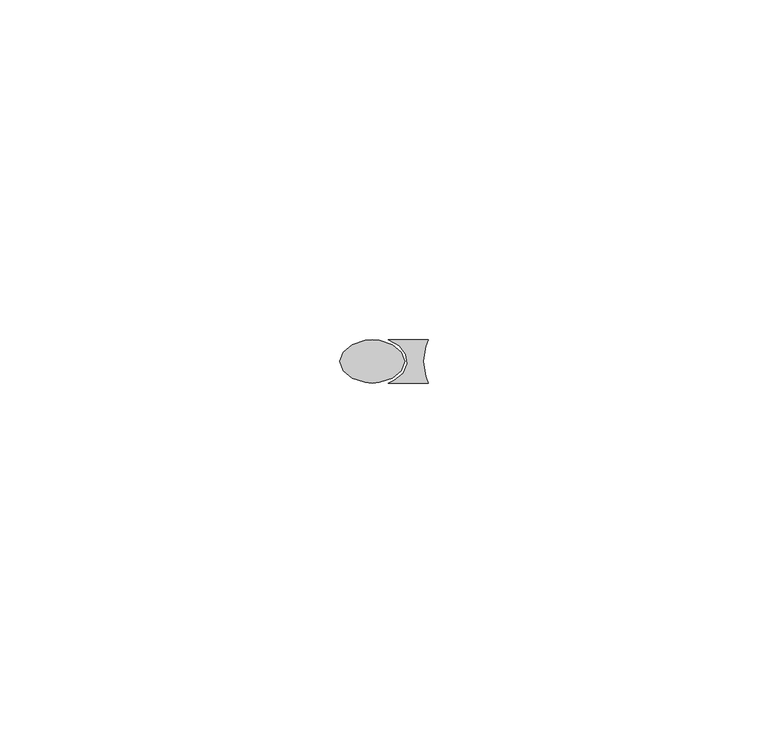
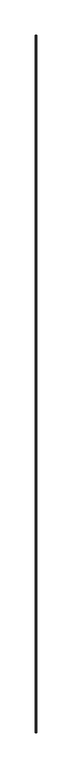
"""IFC4 building model written with IfcOpenShell, lengths in millimetres: proxy geometry, Generic Models 11:Generic Models 1:306267:Generic Models 1:306267 : Generic Models 11:Generic Models 1:306267:300405:Generic Models 1:306267:Generic Models 1:306267 : Generic Models 11:Generic Models 1:306267:300405 : Generic Models 11:Generic Models 1:306267:Generic Models 1:306267 : Generic Models 11:Generic Models 1:306267:300405:35 : Generic Models 11:Generic Models 1:306267:Generic Models 1:306267 : Generic Models 11:Generic Models 1:306267:300405:Generic Models 1:306267:Generic Models 1:306267 : Generic Models 11:Generic Models 1:306267:300405 : Generic Models 11:Generic Models 1:306267:Generic Models 1:306267 : Generic Models 11:Generic Models 1:306267:300405:300182."""

from ifc_helpers import new_model, si_unit, frame, origin, place, context, project, spatial, polyline, outline, extrude, source, transform, mapped, element, save


def generic_models_dcd7ff87(model_context):
    return source(origin(), model_context, "Body", "SweptSolid", [
        extrude(outline(polyline([(573367.5409469, -536525.0496088), (573366.2194528, -536526.1543429), (573364.3098386, -536526.7674241), (573363.2500826, -536526.8470279), (573362.1903267, -536526.7674241), (573360.2807125, -536526.1543429), (573358.9592184, -536525.0496088), (573358.4875826, -536523.6720279), (573358.9592184, -536522.2944471), (573360.2807125, -536521.189713), (573362.1903267, -536520.5766318), (573363.2500826, -536520.4970279), (573364.3098386, -536520.5766318), (573366.2194528, -536521.189713), (573367.5409469, -536522.2944471), (573368.0125826, -536523.6720279), (573367.5409469, -536525.0496088)])), frame((0.0, 0.0, 38.1), z_axis=(0.0, 0.0, 1.0), x_axis=(1.0, 0.0, 0.0)), (0.0, 0.0, 1.0), 6026.3581746),
        extrude(outline(polyline([(573371.1043937, -536521.4627912), (573370.7907076, -536523.6720279), (573371.1043937, -536525.8812647), (573371.4818023, -536526.8470279), (573365.6137102, -536526.8470279), (573366.4739912, -536526.4607104), (573367.7835663, -536525.3772249), (573368.3839199, -536524.0269772), (573368.181132, -536522.6212009), (573367.206927, -536521.3798168), (573365.6137102, -536520.4970279), (573371.4818023, -536520.4970279), (573371.1043937, -536521.4627912)])), frame((0.0, 0.0, 38.1), z_axis=(0.0, 0.0, 1.0), x_axis=(1.0, 0.0, 0.0)), (0.0, 0.0, 1.0), 6024.8878028),
    ])


if __name__ == "__main__":
    model = new_model("IFC4")
    model_context = context("Model", 3, world=origin())
    ifc_project = project(units=[si_unit("LENGTHUNIT", "METRE", prefix="MILLI")], contexts=[model_context])
    site = spatial("IfcSite", under=ifc_project)
    building = spatial("IfcBuilding", under=site)
    placement = place(None, origin())
    generic_models_shape = generic_models_dcd7ff87(model_context)
    element("IfcBuildingElementProxy", 1, Name="Generic Models 11:Generic Models 1:306267:Generic Models 1:306267 : Generic Models 11:Generic Models 1:306267:300405:Generic Models 1:306267:Generic Models 1:306267 : Generic Models 11:Generic Models 1:306267:300405 : Generic Models 11:Generic Models 1:306267:Generic Models 1:306267 : Generic Models 11:Generic Models 1:306267:300405:35 : Generic Models 11:Generic Models 1:306267:Generic Models 1:306267 : Generic Models 11:Generic Models 1:306267:300405:Generic Models 1:306267:Generic Models 1:306267 : Generic Models 11:Generic Models 1:306267:300405 : Generic Models 11:Generic Models 1:306267:Generic Models 1:306267 : Generic Models 11:Generic Models 1:306267:300405:300182", ObjectType="Generic Models 11:Generic Models 1:306267:Generic Models 1:306267 : Generic Models 11:Generic Models 1:306267:300405:Generic Models 1:306267:Generic Models 1:306267 : Generic Models 11:Generic Models 1:306267:300405 : Generic Models 11:Generic Models 1:306267:Generic Models 1:306267 : Generic Models 11:Generic Models 1:306267:300405:35 : Generic Models 11:Generic Models 1:306267:Generic Models 1:306267 : Generic Models 11:Generic Models 1:306267:300405:Generic Models 1:306267:Generic Models 1:306267 : Generic Models 11:Generic Models 1:306267:300405 : Generic Models 11:Generic Models 1:306267:Generic Models 1:306267 : Generic Models 11:Generic Models 1:306267:300405:300182", at=placement, inside=building, context=model_context, shape_type="MappedRepresentation", body=[
        mapped(generic_models_shape, transform((0.0, 0.0, 0.0), x_axis=(1.0, 0.0, 0.0), y_axis=(0.0, 1.0, 0.0), z_axis=(0.0, 0.0, 1.0))),
    ])
    save(model, "model.ifc")

# Revit data of these elements
# Type "Generic Models 11:Generic Models 1:306267:Generic Models 1:306267 : Generic Models 11:Generic Models 1:306267:300405:Generic Models 1:306267:Generic Models 1:306267 : Generic Models 11:Generic Models 1:306267:300405 : Generic Models 11:Generic Models 1:306267:Generic Models 1:306267 : Generic Models 11:Generic Models 1:306267:300405:35 : Generic Models 11:Generic Models 1:306267:Generic Models 1:306267 : Generic Models 11:Generic Models 1:306267:300405:Generic Models 1:306267:Generic Models 1:306267 : Generic Models 11:Generic Models 1:306267:300405 : Generic Models 11:Generic Models 1:306267:Generic Models 1:306267 : Generic Models 11:Generic Models 1:306267:300405:300182"
#   NameOverride = "Generic Models 11:Generic Models 1:306267:Generic Models 1:306267 : Generic Models 11:Generic Models 1:306267:300405:Generic Models 1:306267:Generic Models 1:306267 : Generic Models 11:Generic Models 1:306267:300405 : Generic Models 11:Generic Models 1:306267:Generic Models 1:306267 : Generic Models 11:Generic Models 1:306267:300405:300182"
#   ObjectTypeOverride = "Generic Models 1:306267:Generic Models 1:306267 : Generic Models 11:Generic Models 1:306267:300405 : Generic Models 11:Generic Models 1:306267:Generic Models 1:306267 : Generic Models 11:Generic Models 1:306267:300405"
#   Reference = "Generic Models 1"
#   Tag = "300182"
# Element 1 (IfcBuildingElementProxy, "Generic Models 11:Generic Models 1:306267:Generic Models 1:306267 : Generic Models 11:Generic Models 1:306267:300405:Generic Models 1:306267:Generic Models 1:306267 : Generic Models 11:Generic Models 1:306267:300405 : Generic Models 11:Generic Models 1:306267:Generic Models 1:306267 : Generic Models 11:Generic Models 1:306267:300405:35 : Generic Models 11:Generic Models 1:306267:Generic Models 1:306267 : Generic Models 11:Generic Models 1:306267:300405:Generic Models 1:306267:Generic Models 1:306267 : Generic Models 11:Generic Models 1:306267:300405 : Generic Models 11:Generic Models 1:306267:Generic Models 1:306267 : Generic Models 11:Generic Models 1:306267:300405:300182")
#   Materials on its faces: "SEALANT & BACKER ROD, IF NECESSARY"
# Materials
#   "SEALANT & BACKER ROD, IF NECESSARY": class "Unassigned", colour RGB 120 120 120, transparency 0, Cost = 0
